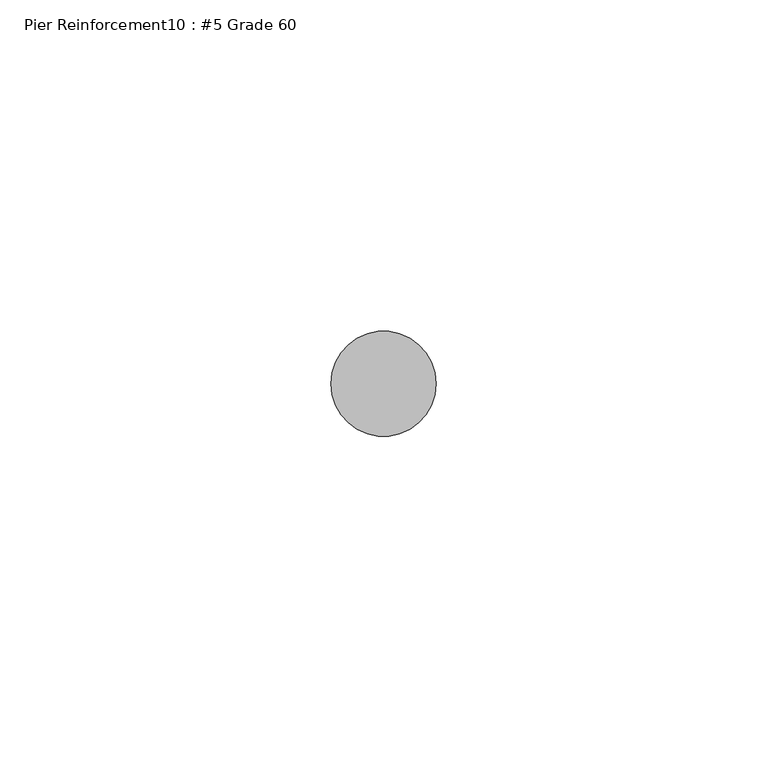
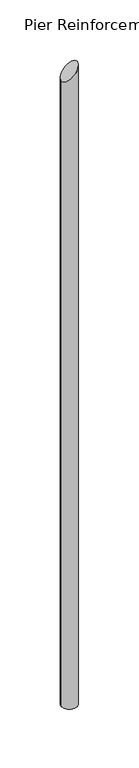
"""IFC4 building model written with IfcOpenShell, lengths in millimetres: proxy geometry, Pier Reinforcement10 : #5 Grade 60."""

from ifc_helpers import new_model, si_unit, frame, origin, place, context, project, spatial, circle_curve, ellipse_curve, source, transform, mapped, element, save
from ifc_brep_helpers import plane_surface, cylinder_surface, advanced_brep


def pier_reinforcement10_5_grade_60_09fa241f(model_context):
    return source(origin(), model_context, "Body", "AdvancedBrep", [
        advanced_brep(
        [(590218.1172365, -534045.8663841, -733.425), (590233.9922365, -534045.8663841, -733.425), (590233.9922365, -534045.8663841, -47.625), (590218.1172365, -534045.8663841, -63.5)],
        [
            (0, 1, circle_curve(frame((590226.0547365, -534045.8663841, -733.425), z_axis=(0.0, 0.0, -1.0), x_axis=(1.0, 0.0, 0.0)), 7.9375)),
            (1, 0, circle_curve(frame((590226.0547365, -534045.8663841, -733.425), z_axis=(0.0, 0.0, -1.0), x_axis=(1.0, 0.0, 0.0)), 7.9375)),
            (1, 2),
            (2, 3, ellipse_curve(frame((590226.0547365, -534045.8663841, -55.5625), z_axis=(0.7071067811865458, 0.0, -0.7071067811865493), x_axis=(0.7071067811865493, 0.0, 0.7071067811865456)), 11.2253202, 7.9375)),
            (3, 0),
            (3, 2, ellipse_curve(frame((590226.0547365, -534045.8663841, -55.5625), z_axis=(0.7071067811865458, 0.0, -0.7071067811865493), x_axis=(0.7071067811865493, 0.0, 0.7071067811865456)), 11.2253202, 7.9375)),
        ],
        [
            plane_surface(frame((590233.9922365, -534045.8663841, -733.425), z_axis=(0.0, 0.0, -1.0), x_axis=(0.0, -1.0, 0.0))),
            cylinder_surface(frame((590226.0547365, -534045.8663841, -733.425), z_axis=(0.0, 0.0, 1.0), x_axis=(1.0, 0.0, 0.0)), 7.9375),
            plane_surface(frame((590233.9922365, -534020.4663841, -47.625), z_axis=(-0.7071067811865458, 0.0, 0.7071067811865493), x_axis=(0.0, -1.0, 0.0))),
        ],
        [
            (0, [[1, 2]]),
            (1, [[-2, 3, 4, 5]]),
            (1, [[-1, -5, 6, -3]]),
            (2, [[-4, -6]]),
        ],
    ),
    ])


if __name__ == "__main__":
    model = new_model("IFC4")
    model_context = context("Model", 3, world=origin())
    ifc_project = project(units=[si_unit("LENGTHUNIT", "METRE", prefix="MILLI")], contexts=[model_context])
    site = spatial("IfcSite", under=ifc_project)
    building = spatial("IfcBuilding", under=site)
    placement = place(None, origin())
    pier_reinforcement10_5_grade_60_shape = pier_reinforcement10_5_grade_60_09fa241f(model_context)
    element("IfcBuildingElementProxy", 1, Name="Pier Reinforcement10 : #5 Grade 60", ObjectType="Pier Reinforcement10 : #5 Grade 60", at=placement, inside=building, context=model_context, shape_type="MappedRepresentation", body=[
        mapped(pier_reinforcement10_5_grade_60_shape, transform((0.0, 0.0, 0.0), x_axis=(1.0, 0.0, 0.0), y_axis=(0.0, 1.0, 0.0), z_axis=(0.0, 0.0, 1.0))),
    ])
    save(model, "model.ifc")

# Revit data of these elements
# Element 1 (IfcBuildingElementProxy, "Pier Reinforcement10 : #5 Grade 60")
#   Materials on its faces: "#5 GR. 60 BEND 24\"x24\""
# Materials
#   "#5 GR. 60 BEND 24\"x24\"": class "Generic", colour RGB 84 83 81, transparency 0, Cost = 0
